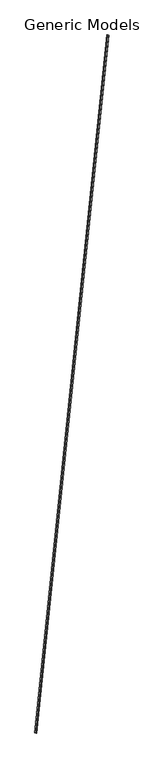
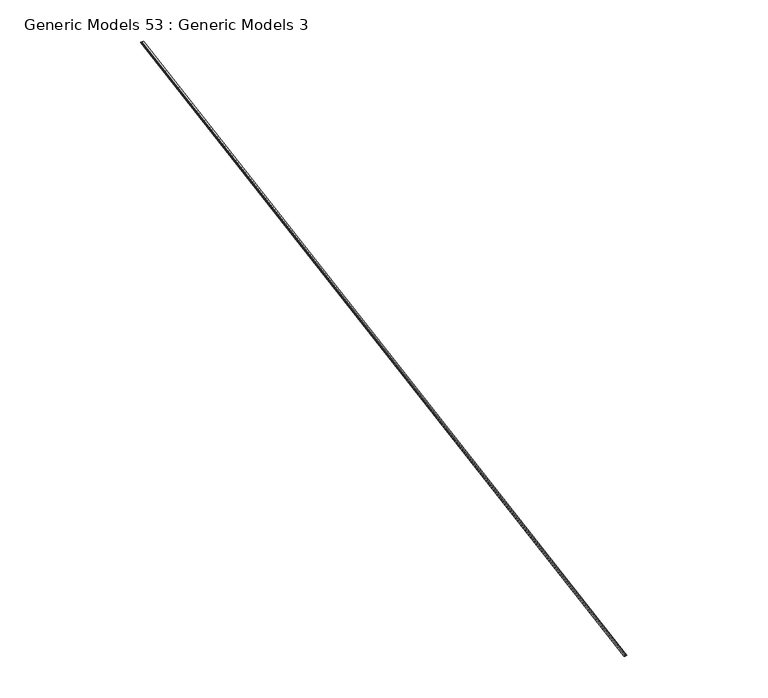
"""IFC4 building model written with IfcOpenShell, lengths in millimetres: proxy geometry, Generic Models 53 : Generic Models 3."""

from ifc_helpers import new_model, si_unit, frame, origin, place, context, project, spatial, polyline, outline, extrude, source, transform, mapped, element, save


def generic_models_53_generic_models_3_9d4f647c(model_context):
    return source(origin(), model_context, "Body", "SweptSolid", [
        extrude(outline(polyline([(19.6759914, 0.0), (28.4072055, 6.9504923), (45.7208472, 6.9504922), (45.7208472, 5.3629922), (28.9619207, 5.3629922), (20.2307067, -1.5875), (1.9622579, -1.5875001), (1.9622579, 0.0), (19.6759914, 0.0)])), frame((35178.2535324, 40710.3080382, 272203.8217466), z_axis=(-0.10293344407674773, -0.9946674410191907, 0.006433340254794668), x_axis=(0.9927304042422549, -0.1031342900122695, -0.062045650263933584)), (0.0, 0.0, 1.0), 15089.019704),
    ])


if __name__ == "__main__":
    model = new_model("IFC4")
    model_context = context("Model", 3, world=origin())
    ifc_project = project(units=[si_unit("LENGTHUNIT", "METRE", prefix="MILLI")], contexts=[model_context])
    site = spatial("IfcSite", under=ifc_project)
    building = spatial("IfcBuilding", under=site)
    placement = place(None, origin())
    generic_models_53_generic_models_3_shape = generic_models_53_generic_models_3_9d4f647c(model_context)
    element("IfcBuildingElementProxy", 1, Name="Generic Models 53 : Generic Models 3", ObjectType="Generic Models 53 : Generic Models 3", at=placement, inside=building, context=model_context, shape_type="MappedRepresentation", body=[
        mapped(generic_models_53_generic_models_3_shape, transform((0.0, 0.0, 0.0), x_axis=(1.0, 0.0, 0.0), y_axis=(0.0, 1.0, 0.0), z_axis=(0.0, 0.0, 1.0))),
    ])
    save(model, "model.ifc")

# Revit data of these elements
# Element 1 (IfcBuildingElementProxy, "Generic Models 53 : Generic Models 3")
#   Materials on its faces: "GALV. STANDING SEAM METAL ROOF"
# Materials
#   "GALV. STANDING SEAM METAL ROOF": class "Unassigned", colour RGB 228 228 228, transparency 0, Comments = "Rendering appearance not upgraded ", Description = "Standing Metal Seam Roof", Cost = 0
